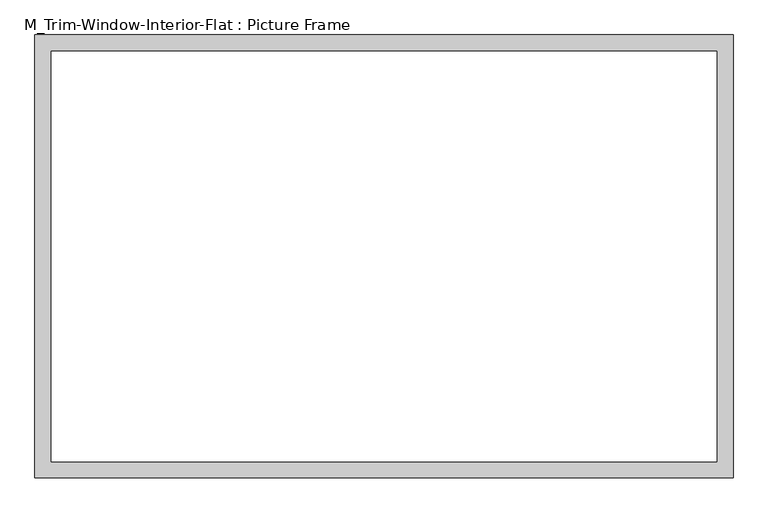
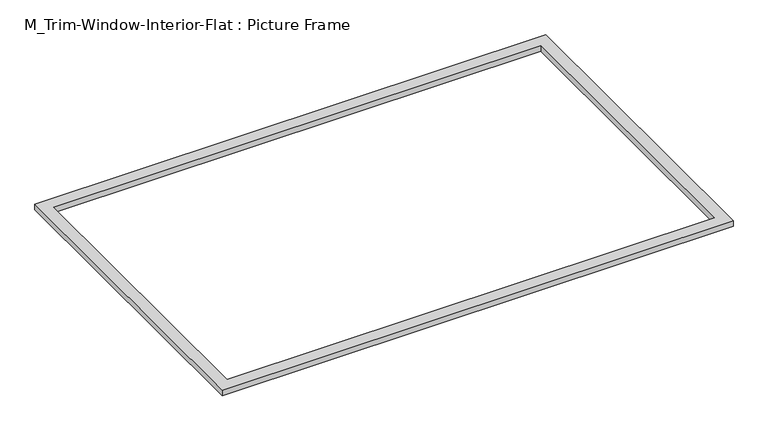
"""IFC4 building model written with IfcOpenShell, lengths in millimetres: proxy geometry, M_Trim-Window-Interior-Flat : Picture Frame."""

from ifc_helpers import new_model, si_unit, origin, origin_with_axes, place, context, project, spatial, polyline, outline, extrude, source, transform, mapped, element, save


def m_trim_window_interior_flat_picture_frame_cdca9661(model_context):
    return source(origin(), model_context, "Body", "SweptSolid", [
        extrude(outline(polyline([(1297.3, 47.3), (1297.3, -1598.1), (-1297.3, -1598.1), (-1297.3, 47.3), (1297.3, 47.3)]), holes=[polyline([(1237.3, -12.7), (-1237.3, -12.7), (-1237.3, -1538.1), (1237.3, -1538.1), (1237.3, -12.7)])]), origin_with_axes(), (0.0, 0.0, 1.0), 30.0),
    ])


if __name__ == "__main__":
    model = new_model("IFC4")
    model_context = context("Model", 3, world=origin())
    ifc_project = project(units=[si_unit("LENGTHUNIT", "METRE", prefix="MILLI")], contexts=[model_context])
    site = spatial("IfcSite", under=ifc_project)
    building = spatial("IfcBuilding", under=site)
    placement = place(None, origin())
    m_trim_window_interior_flat_picture_frame_shape = m_trim_window_interior_flat_picture_frame_cdca9661(model_context)
    element("IfcBuildingElementProxy", 1, Name="M_Trim-Window-Interior-Flat : Picture Frame", ObjectType="M_Trim-Window-Interior-Flat : Picture Frame", at=placement, inside=building, context=model_context, shape_type="MappedRepresentation", body=[
        mapped(m_trim_window_interior_flat_picture_frame_shape, transform((0.0, 0.0, 0.0), x_axis=(1.0, 0.0, 0.0), y_axis=(0.0, 1.0, 0.0), z_axis=(0.0, 0.0, 1.0))),
    ])
    save(model, "model.ifc")

# Revit data of these elements
# Type "M_Trim-Window-Interior-Flat : Picture Frame"
#   Trim Thickness_Picture Frame = 30 mm
#   Trim Width = 60 mm
#   Trim Thickness_with Sill = 20 mm
#   Sill Thickness = 30 mm
#   Opening Width [instance default] = 600 mm
#   Opening Height [instance default] = 900 mm
#   Default Elevation = 1200 mm
#   Sill = no
#   Picture Frame = yes
#   Trim Material [instance default] = none
# Element 1 (IfcBuildingElementProxy, "M_Trim-Window-Interior-Flat : Picture Frame")
#   Opening Width = 2500 mm
#   Opening Height = 1550.8 mm
#   Trim Material = Wood - Stained
#   Materials on its faces: "Wood - Stained"
# Materials
#   "Wood - Stained": class "Wood", colour RGB 227 170 128, transparency 0, Cost = 0
